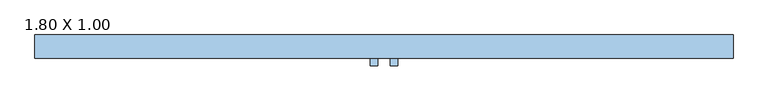
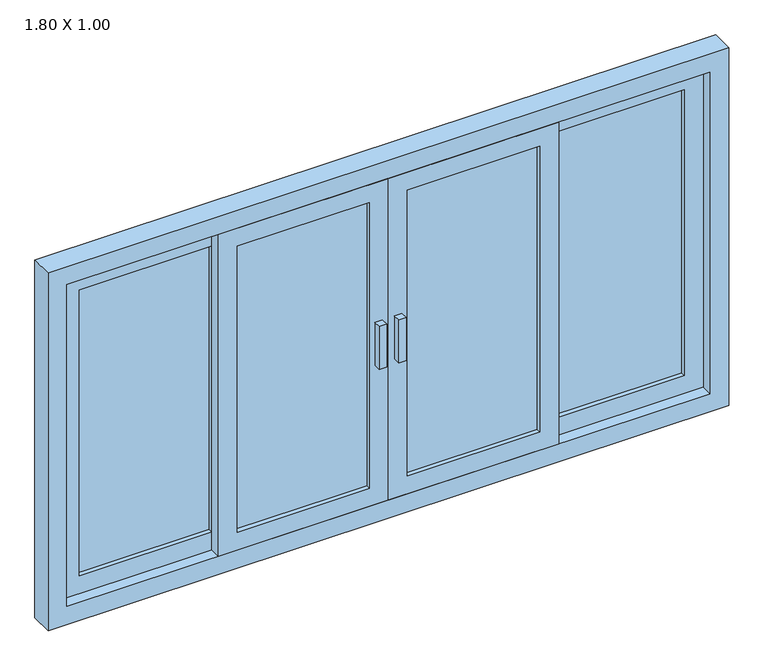
"""IFC4 building model written with IfcOpenShell, lengths in millimetres: window geometry, JANELA_DE_CORRER_4 FOLHAS_VIDRO : 1.80 X 1.00."""

from ifc_helpers import new_model, si_unit, frame, origin, place, context, project, spatial, polyline, outline, extrude, source, transform, mapped, element, save


def window_1_80_x_1_00_39fb8669(model_context):
    return source(origin(), model_context, "Body", "SweptSolid", [
        extrude(outline(polyline([(800.0, 17.5), (800.0, 12.5), (450.0, 12.5), (450.0, 17.5), (800.0, 17.5)])), frame((0.0, 0.0, 1100.0), z_axis=(0.0, 0.0, 1.0), x_axis=(1.0, 0.0, 0.0)), (0.0, 0.0, 1.0), 800.0),
        extrude(outline(polyline([(1950.0, 850.0), (1950.0, 400.0), (1050.0, 400.0), (1050.0, 850.0), (1950.0, 850.0)]), holes=[polyline([(1900.0, 800.0), (1100.0, 800.0), (1100.0, 450.0), (1900.0, 450.0), (1900.0, 800.0)])]), frame((0.0, 0.0, 0.0), z_axis=(0.0, 1.0, 0.0), x_axis=(0.0, 0.0, 1.0)), (0.0, 0.0, 1.0), 30.0),
        extrude(outline(polyline([(400.0, -12.5), (400.0, -17.5), (50.0, -17.5), (50.0, -12.5), (400.0, -12.5)])), frame((0.0, 0.0, 1100.0), z_axis=(0.0, 0.0, 1.0), x_axis=(1.0, 0.0, 0.0)), (0.0, 0.0, 1.0), 800.0),
        extrude(outline(polyline([(1950.0, 450.0), (1950.0, 0.0), (1050.0, 0.0), (1050.0, 450.0), (1950.0, 450.0)]), holes=[polyline([(1900.0, 400.0), (1100.0, 400.0), (1100.0, 50.0), (1900.0, 50.0), (1900.0, 400.0)])]), frame((0.0, -30.0, 0.0), z_axis=(0.0, 1.0, 0.0), x_axis=(0.0, 0.0, 1.0)), (0.0, 0.0, 1.0), 30.0),
        extrude(outline(polyline([(-50.0, -12.5), (-50.0, -17.5), (-400.0, -17.5), (-400.0, -12.5), (-50.0, -12.5)])), frame((0.0, 0.0, 1100.0), z_axis=(0.0, 0.0, 1.0), x_axis=(1.0, 0.0, 0.0)), (0.0, 0.0, 1.0), 800.0),
        extrude(outline(polyline([(1950.0, 0.0), (1950.0, -450.0), (1050.0, -450.0), (1050.0, 0.0), (1950.0, 0.0)]), holes=[polyline([(1900.0, -50.0), (1100.0, -50.0), (1100.0, -400.0), (1900.0, -400.0), (1900.0, -50.0)])]), frame((0.0, -30.0, 0.0), z_axis=(0.0, 1.0, 0.0), x_axis=(0.0, 0.0, 1.0)), (0.0, 0.0, 1.0), 30.0),
        extrude(outline(polyline([(-450.0, 17.5), (-450.0, 12.5), (-800.0, 12.5), (-800.0, 17.5), (-450.0, 17.5)])), frame((0.0, 0.0, 1100.0), z_axis=(0.0, 0.0, 1.0), x_axis=(1.0, 0.0, 0.0)), (0.0, 0.0, 1.0), 800.0),
        extrude(outline(polyline([(1950.0, -400.0), (1950.0, -850.0), (1050.0, -850.0), (1050.0, -400.0), (1950.0, -400.0)]), holes=[polyline([(1900.0, -450.0), (1100.0, -450.0), (1100.0, -800.0), (1900.0, -800.0), (1900.0, -450.0)])]), frame((0.0, 0.0, 0.0), z_axis=(0.0, 1.0, 0.0), x_axis=(0.0, 0.0, 1.0)), (0.0, 0.0, 1.0), 30.0),
        extrude(outline(polyline([(15.9492003, -30.0), (35.9492003, -30.0), (35.9492003, -50.0), (15.9492003, -50.0), (15.9492003, -30.0)])), frame((0.0, 0.0, 1440.0), z_axis=(0.0, 0.0, 1.0), x_axis=(1.0, 0.0, 0.0)), (0.0, 0.0, 1.0), 120.0),
        extrude(outline(polyline([(-35.9492003, -30.0), (-15.9492003, -30.0), (-15.9492003, -50.0), (-35.9492003, -50.0), (-35.9492003, -30.0)])), frame((0.0, 0.0, 1440.0), z_axis=(0.0, 0.0, 1.0), x_axis=(1.0, 0.0, 0.0)), (0.0, 0.0, 1.0), 120.0),
        extrude(outline(polyline([(1000.0, -900.0), (1000.0, 900.0), (2000.0, 900.0), (2000.0, -900.0), (1000.0, -900.0)]), holes=[polyline([(1950.0, -850.0), (1950.0, 850.0), (1050.0, 850.0), (1050.0, -850.0), (1950.0, -850.0)])]), frame((0.0, -30.0, 0.0), z_axis=(0.0, 1.0, 0.0), x_axis=(0.0, 0.0, 1.0)), (0.0, 0.0, 1.0), 60.0),
    ])


if __name__ == "__main__":
    model = new_model("IFC4")
    model_context = context("Model", 3, world=origin())
    ifc_project = project(units=[si_unit("LENGTHUNIT", "METRE", prefix="MILLI")], contexts=[model_context])
    site = spatial("IfcSite", under=ifc_project)
    building = spatial("IfcBuilding", under=site)
    placement = place(None, origin())
    window_1_80_x_1_00_shape = window_1_80_x_1_00_39fb8669(model_context)
    element("IfcWindow", 1, ObjectType="JANELA_DE_CORRER_4 FOLHAS_VIDRO : 1.80 X 1.00", at=placement, inside=building, context=model_context, shape_type="MappedRepresentation", body=[
        mapped(window_1_80_x_1_00_shape, transform((0.0, 0.0, 0.0), x_axis=(1.0, 0.0, 0.0), y_axis=(0.0, 1.0, 0.0), z_axis=(0.0, 0.0, 1.0))),
    ])
    save(model, "model.ifc")

# Revit data of these elements
# Type "JANELA_DE_CORRER_4 FOLHAS_VIDRO : 1.80 X 1.00"
#   Type Mark = "J4"
#   Analytic Construction = "<Nenhum>"
#   Largura moldura = 0.06 m
#   Largura janela = 1.70 m
#   Largura esquadria = 0.05 m
#   Largura do painel = 0.45 m
#   Largura da moldura do painel = 0.05 m
#   Espessura painel = 0.03 m
#   Espessura moldura = 0.03 m
#   Altura janela = 0.90 m
#   Height = 1.00 m
#   Altura-padrão do peitoril = 1.00 m
#   Width = 1.80 m
#   Puxadores [instance default] = yes
#   Moldura interna [instance default] = yes
#   Moldura externa [instance default] = yes
#   Tipo de vidro = .VIDRO
#   Material puxadores = .ALUMÍNIO COM PINTURA ELETROSTÁTICA BRANCA
#   Material moldura = .ALUMÍNIO COM PINTURA ELETROSTÁTICA BRANCA
#   Material da esquadria = .ALUMÍNIO COM PINTURA ELETROSTÁTICA BRANCA
#   Wall Closure = (empty or 0)
# Element 1 (IfcWindow, "JANELA_DE_CORRER_4 FOLHAS_VIDRO : 1.80 X 1.00")
#   Moldura interna = no
#   Moldura externa = no
#   Materials on its faces: ".ALUMÍNIO COM PINTURA ELETROSTÁTICA BRANCA", ".VIDRO"
# Materials
#   ".VIDRO": class "Genérico", colour RGB 198 236 255, transparency 0.95, Cost = 0
#   ".ALUMÍNIO COM PINTURA ELETROSTÁTICA BRANCA": class "CC_METAIS", colour RGB 241 241 241, transparency 0, Cost = 0
